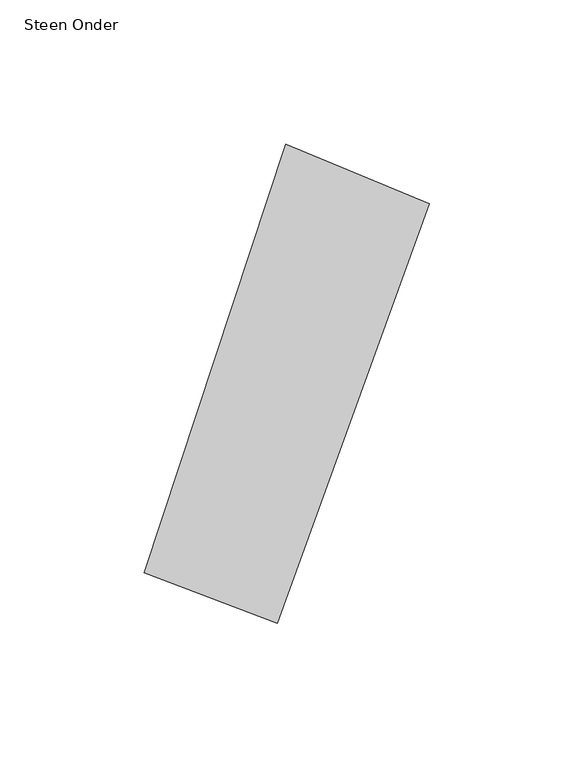
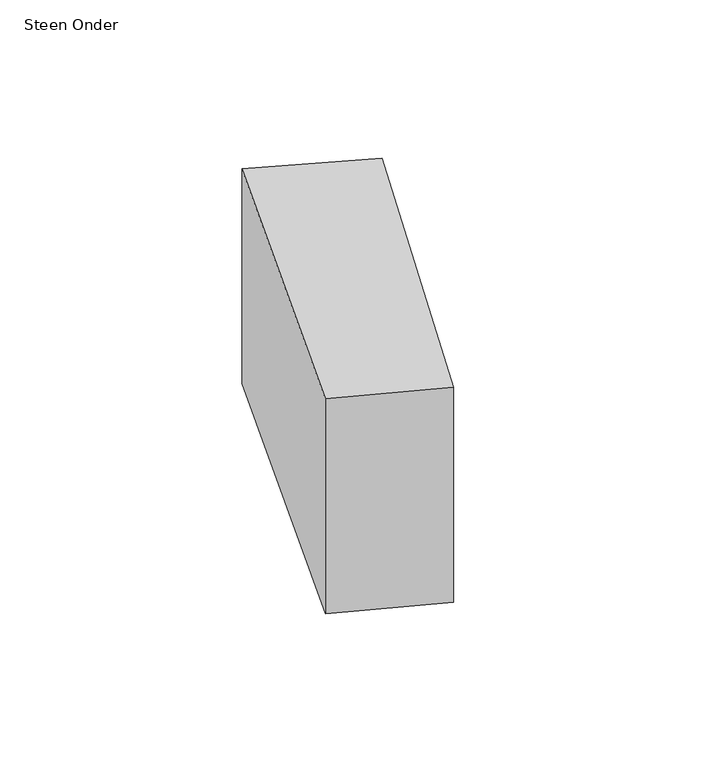
"""IFC4 building model written with IfcOpenShell, lengths in millimetres: proxy geometry, 00_GMA_steen_versie_4 : Steen Onder."""

from ifc_helpers import new_model, si_unit, origin, origin_with_axes, place, context, project, spatial, polyline, outline, extrude, source, transform, mapped, element, save


def steen_onder_780e947e(model_context):
    return source(origin(), model_context, "Body", "SweptSolid", [
        extrude(outline(polyline([(126.390494, 140.8204635), (73.8168995, -4.3922163), (27.7812432, 13.2320641), (76.6162622, 161.3868929), (126.390494, 140.8204635)])), origin_with_axes(), (0.0, 0.0, 1.0), 100.0),
    ])


if __name__ == "__main__":
    model = new_model("IFC4")
    model_context = context("Model", 3, world=origin())
    ifc_project = project(units=[si_unit("LENGTHUNIT", "METRE", prefix="MILLI")], contexts=[model_context])
    site = spatial("IfcSite", under=ifc_project)
    building = spatial("IfcBuilding", under=site)
    placement = place(None, origin())
    steen_onder_shape = steen_onder_780e947e(model_context)
    element("IfcBuildingElementProxy", 1, Name="00_GMA_steen_versie_4 : Steen Onder", ObjectType="00_GMA_steen_versie_4 : Steen Onder", at=placement, inside=building, context=model_context, shape_type="MappedRepresentation", body=[
        mapped(steen_onder_shape, transform((0.0, 0.0, 0.0), x_axis=(1.0, 0.0, 0.0), y_axis=(0.0, 1.0, 0.0), z_axis=(0.0, 0.0, 1.0))),
    ])
    save(model, "model.ifc")

# Revit data of these elements
# Type "00_GMA_steen_versie_4 : Steen Onder"
#   StootVoegHalfBoven [instance default] = 5 mm
#   StootVoegHalf [instance default] = 5 mm
#   StootVoegBreedteOnder = 10 mm
#   StootVoegBreedteBoven = 10 mm
#   Steendikte = 100 mm
#   LintVoegOnderHalf = 0 mm
#   LintVoegOnder = 0 mm
#   LintVoegBovenHalf = 5 mm
#   LintVoegBoven = 10 mm
#   materiaal = none
#   MateriaalVoeg = none
#   Default Elevation = 0
